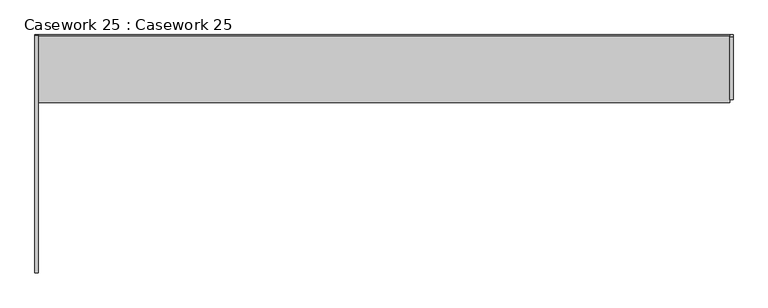
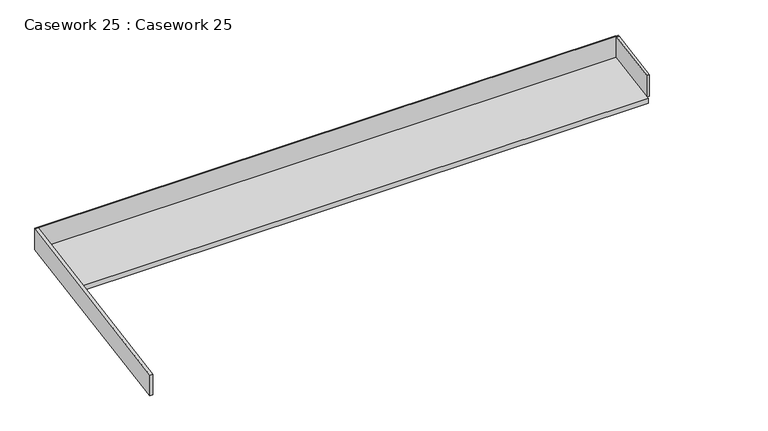
"""IFC4 building model written with IfcOpenShell, lengths in millimetres: furniture geometry, Casework 25 : Casework 25."""

from ifc_helpers import new_model, si_unit, frame, origin, place, context, project, spatial, polyline, outline, extrude, source, transform, mapped, element, save


def casework_25_casework_25_bbe771a2(model_context):
    return source(origin(), model_context, "Body", "SweptSolid", [
        extrude(outline(polyline([(287433.899125, 6477.1627257), (281718.899125, 5511.2472328), (281718.899125, 6139.0579051), (287408.499125, 7136.519522), (287433.899125, 7136.519522), (287433.899125, 6477.1627257)])), frame((-58805.9633954, 0.0, 0.0), z_axis=(1.0, 0.0, 0.0), x_axis=(0.0, 1.0, 0.0)), (0.0, 0.0, 1.0), 79.0707348),
        extrude(outline(polyline([(287433.899125, 6477.1627257), (285884.499125, 6215.2923032), (285884.499125, 6873.7207742), (287391.604592, 7128.8297726), (287433.899125, 7128.8297726), (287433.899125, 6477.1627257)])), frame((-42133.813494, 0.0, 0.0), z_axis=(1.0, 0.0, 0.0), x_axis=(0.0, 1.0, 0.0)), (0.0, 0.0, 1.0), 74.7639834),
        extrude(outline(polyline([(287408.499125, 6498.6299987), (287408.499125, 7136.519522), (287433.899125, 7136.519522), (287433.899125, 6477.1627257), (285831.580213, 6206.3482617), (285831.580213, 6075.4155347), (285806.180213, 6075.4155347), (285806.180213, 6227.8155347), (287408.499125, 6498.6299987)])), frame((-58726.8926606, 0.0, 0.0), z_axis=(1.0, 0.0, 0.0), x_axis=(0.0, 1.0, 0.0)), (0.0, 0.0, 1.0), 16593.0791667),
    ])


if __name__ == "__main__":
    model = new_model("IFC4")
    model_context = context("Model", 3, world=origin())
    ifc_project = project(units=[si_unit("LENGTHUNIT", "METRE", prefix="MILLI")], contexts=[model_context])
    site = spatial("IfcSite", under=ifc_project)
    building = spatial("IfcBuilding", under=site)
    placement = place(None, origin())
    casework_25_casework_25_shape = casework_25_casework_25_bbe771a2(model_context)
    element("IfcFurniture", 1, ObjectType="Casework 25 : Casework 25", at=placement, inside=building, context=model_context, shape_type="MappedRepresentation", body=[
        mapped(casework_25_casework_25_shape, transform((0.0, 0.0, 0.0), x_axis=(1.0, 0.0, 0.0), y_axis=(0.0, 1.0, 0.0), z_axis=(0.0, 0.0, 1.0))),
    ])
    save(model, "model.ifc")

# Revit data of these elements
# Element 1 (IfcFurniture, "Casework 25 : Casework 25")
#   Materials on its faces: "Dark metal"
# Materials
#   "Dark metal": class "Generic", colour RGB 44 29 29, transparency 0, Cost = 0
